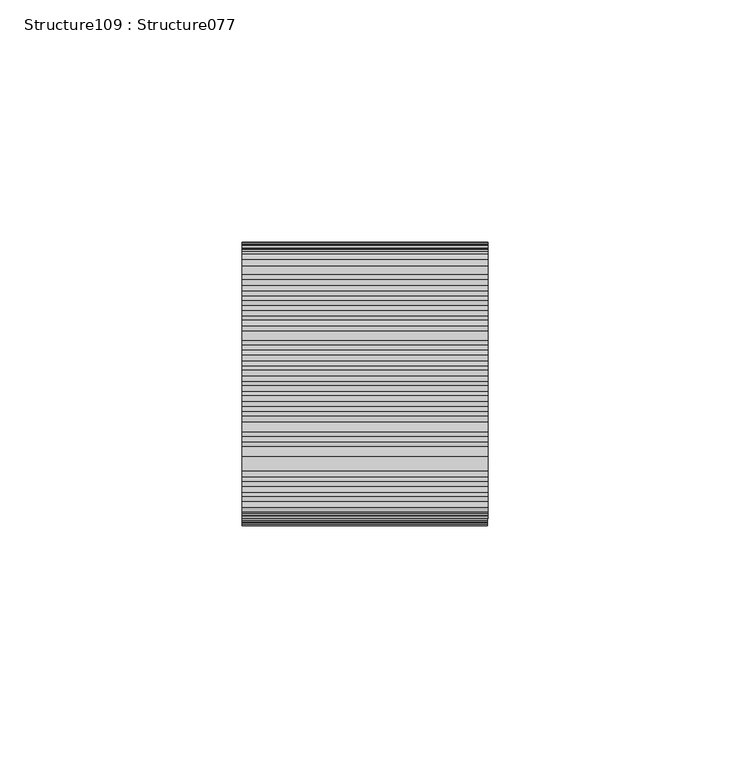
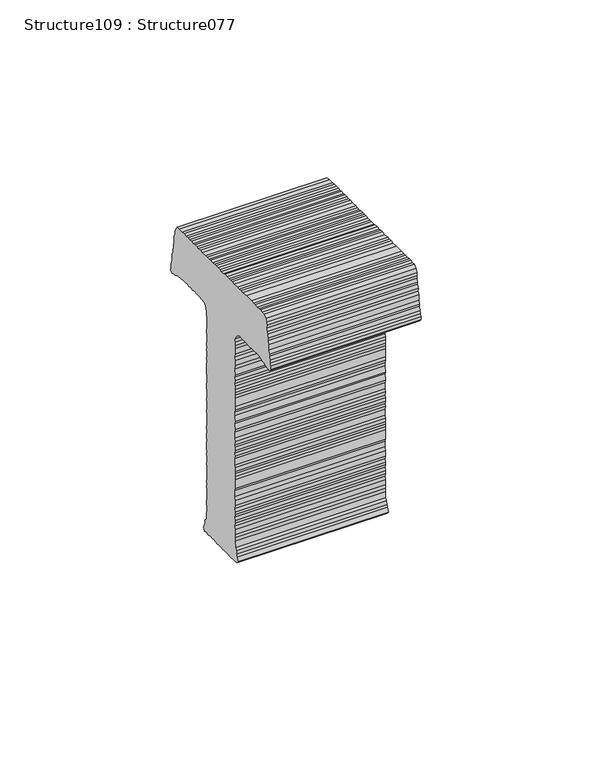
"""IFC4 building model written with IfcOpenShell, lengths in millimetres: proxy geometry, Structure109 : Structure077."""

from ifc_helpers import new_model, si_unit, frame, origin, place, context, project, spatial, polyline, outline, extrude, source, transform, mapped, element, save


def structure109_structure077_04282f25(model_context):
    return source(origin(), model_context, "Body", "SweptSolid", [
        extrude(outline(polyline([(1.289959, 0.0), (2.4826398, -0.634609), (3.3164572, -1.0932807), (3.9580093, -1.9186696), (4.9710555, -2.555887), (5.6151661, -3.0146845), (6.7250256, -3.5599982), (7.3660728, -4.3848855), (8.472829, -4.7530822), (9.8531305, -6.1242604), (10.9554405, -6.6690959), (11.5100349, -7.2200247), (12.6129687, -7.9530557), (13.4427489, -8.4082184), (14.2725291, -8.8633811), (15.1037896, -9.6891473), (15.1944421, -10.698522), (14.1870202, -11.5298818), (13.2730325, -12.0849252), (12.3559164, -12.4553038), (11.5300277, -13.0978639), (10.7973441, -13.4709018), (9.0493141, -14.4858701), (8.3217174, -15.4066268), (7.7726498, -16.1431226), (6.9457747, -16.7917245), (6.1253802, -17.8013525), (5.4844272, -18.4465702), (4.5633947, -19.001637), (3.7416407, -19.8288587), (3.2853709, -20.4764833), (2.2751721, -21.3050846), (1.543944, -22.0411781), (1.0973356, -24.1608888), (1.6488975, -25.9977611), (2.4780178, -26.6333239), (3.3998042, -27.367962), (4.0491583, -28.1940798), (5.4307221, -29.5665119), (6.2585694, -30.5769647), (7.1799825, -31.1231547), (8.4699132, -32.4045593), (9.2069822, -33.5058896), (10.7732057, -34.8736837), (11.2367929, -35.5222839), (12.2485769, -36.1582475), (12.8912362, -37.1657919), (13.6346844, -37.5351933), (14.4614986, -38.5375982), (15.2886229, -39.1781998), (15.9366173, -39.8219112), (16.6745753, -40.7360473), (18.7947568, -42.8422151), (19.7140189, -43.5743455), (20.1741694, -44.4005875), (21.0044202, -45.2253507), (22.6654609, -46.5062796), (23.0352406, -47.2427481), (24.6922424, -48.5196647), (25.2470551, -49.4399433), (26.8111276, -50.9936778), (27.6447916, -51.6337544), (28.4723865, -52.6439564), (29.1169786, -53.0962108), (30.038765, -53.8308488), (30.5895388, -54.7471151), (31.332832, -55.2974182), (31.9756463, -56.1240609), (33.5424955, -57.6805538), (34.2814973, -58.2265939), (35.2908779, -59.0482471), (35.8480941, -59.782836), (36.4905351, -60.4210307), (37.3206885, -61.0646414), (39.6269128, -63.3556224), (40.0845389, -64.1793567), (41.5610173, -65.646076), (42.5766853, -66.4669536), (43.9585014, -67.8396364), (44.6000535, -68.6650253), (45.523991, -69.2137229), (46.1692087, -69.854676), (46.7214971, -70.7724469), (47.6467942, -71.5035509), (48.3821304, -72.2340268), (49.0277214, -73.0634279), (49.9502418, -73.7917735), (51.2404249, -75.0734289), (52.0662869, -75.7127767), (52.8989071, -76.7209493), (54.5549225, -78.0039076), (55.4788926, -78.1830031), (56.4913023, -79.0076656), (57.2264202, -79.3687917), (58.6082305, -79.8291689), (58.7026461, -80.8352603), (57.9676565, -81.5751403), (57.3267991, -82.4010073), (56.50542, -83.4171802), (55.9549928, -83.9712697), (55.1291024, -84.6133267), (53.6628846, -86.0893001), (52.935542, -87.0108108), (52.1058902, -87.6566542), (51.2838854, -88.4841283), (50.7378453, -89.2231301), (49.9083484, -89.6880719), (49.1771203, -90.4241653), (48.4419756, -91.3449471), (47.7141624, -91.8968573), (47.1679673, -92.8167607), (46.0633822, -93.558621), (45.4222741, -94.3847406), (44.2272873, -94.1169737), (43.8574103, -93.1993527), (43.5804608, -92.0044109), (42.6585769, -91.0886203), (42.5601224, -90.0785165), (40.9893892, -88.3371098), (40.6233961, -87.6044028), (39.7960195, -86.9635506), (38.8722369, -86.2339511), (38.2270192, -85.592998), (37.4927269, -84.4944262), (36.8448298, -84.0318672), (36.0162486, -83.0277069), (35.3672443, -82.3829923), (34.4470933, -81.8380561), (33.8989413, -81.1054499), (33.0652772, -80.4653733), (32.5145035, -79.549107), (29.3755039, -76.4308552), (28.6416482, -76.0709829), (27.9988339, -75.2443402), (27.0731636, -74.3247882), (26.2422762, -73.6874699), (25.6009766, -72.8623318), (24.9520932, -72.4058145), (23.3854964, -70.8495724), (22.7428371, -69.8420279), (21.821424, -69.2958379), (21.1736819, -68.6523772), (20.5308676, -67.8257344), (19.6096094, -67.0986426), (18.3179459, -65.4463837), (17.5794256, -64.8938004), (16.7509417, -64.0707925), (16.2921742, -63.4340016), (15.090056, -62.6089619), (14.6310127, -61.9648754), (13.9887267, -61.1457791), (12.9725304, -60.3173552), (12.3279384, -59.8651009), (11.6784635, -58.8507858), (10.945749, -58.30397), (10.2991717, -57.4806107), (9.280572, -56.8378764), (8.4536027, -56.0163732), (7.9067128, -55.2850208), (7.2560966, -54.4576492), (6.6108788, -53.8166961), (5.6869413, -53.2679984), (3.4748744, -51.0705525), (2.740582, -49.9719806), (1.9113067, -49.5173194), (1.3560867, -48.7776919), (0.620498, -48.0469653), (-0.2129136, -47.4071394), (-0.7654545, -46.4891177), (-1.6823238, -45.9474415), (-2.3317988, -44.9331264), (-3.1594278, -44.2920234), (-3.8950165, -43.5612967), (-4.8203136, -42.8301927), (-6.1079382, -41.181946), (-6.9378391, -40.538586), (-7.3981213, -39.9002905), (-8.3199077, -39.1656525), (-9.1505426, -38.528585), (-9.7955079, -37.8878827), (-11.5384176, -36.8807156), (-12.4611829, -37.0649281), (-13.8384528, -37.8980173), (-14.8461289, -38.7286231), (-15.3965561, -39.2827127), (-16.0358988, -40.1100843), (-16.9497891, -40.8462803), (-17.5928932, -41.6774383), (-18.6009408, -42.3200993), (-19.0556003, -43.1498778), (-19.8825962, -43.6102823), (-20.612344, -44.7169794), (-21.3486932, -45.2744531), (-23.1741727, -47.6684522), (-23.7231446, -48.5855974), (-24.1776816, -49.6040764), (-24.6342272, -50.2444054), (-25.1856026, -51.3472402), (-26.2867062, -51.166216), (-26.7507747, -50.5241591), (-27.5782488, -49.7021543), (-28.1285194, -48.7858863), (-28.5969769, -47.9584139), (-29.4239461, -47.1369107), (-30.1573836, -46.2202437), (-30.4442844, -45.2110164), (-30.9911743, -44.479664), (-31.5499051, -43.7435706), (-32.286756, -43.0115901), (-32.7467531, -42.0039433), (-33.6726759, -41.0841405), (-34.3148645, -40.4461966), (-34.684839, -39.3474231), (-35.5160995, -38.5216569), (-35.9848061, -36.4049811), (-35.1593865, -35.3933237), (-33.877731, -34.1031405), (-33.2381375, -33.2755165), (-32.3207366, -32.5357865), (-31.5906172, -31.6170343), (-30.7675037, -30.972219), (-30.2149253, -30.232189), (-29.3014407, -29.6771472), (-28.7522182, -28.7597496), (-27.9267027, -27.9287414), (-27.1977806, -27.5594901), (-26.4604849, -26.452768), (-25.5467496, -25.8974738), (-24.2649393, -24.4263889), (-23.533866, -23.8711972), (-22.7988764, -23.1313173), (-22.2496538, -22.2139197), (-21.3360143, -21.4779761), (-20.6929102, -20.646818), (-20.0522078, -20.0018527), (-19.1383176, -19.2656567), (-18.3128021, -18.4346486), (-17.6722547, -17.970585), (-16.7597241, -17.0519827), (-16.3880425, -16.3133074), (-15.4757627, -15.3949576), (-14.6488875, -14.7463557), (-14.009294, -13.9187316), (-13.3685917, -13.2737663), (-12.3608199, -12.6238099), (-11.0803691, -10.9703188), (-10.3440199, -10.4128451), (-9.6141513, -9.4943453), (-8.7909419, -9.0301793), (-7.5104911, -7.3766882), (-5.3998096, -5.2519629), (-4.3918828, -4.4211047), (-3.7546911, -3.7796734), (-2.9293306, -3.1295671), (-2.1976967, -2.2123194), (-1.6488799, -1.476076), (-0.7316338, -0.9172476), (0.0, 0.0), (1.289959, 0.0)])), frame((-56111.5642738, 291173.858936, -276.594816), z_axis=(-0.9999998917542983, 0.0004652863545059615, 0.0), x_axis=(-0.0003279144188290442, -0.7047582207414732, -0.7094474911996285)), (0.0, 0.0, 1.0), 50.8),
    ])


if __name__ == "__main__":
    model = new_model("IFC4")
    model_context = context("Model", 3, world=origin())
    ifc_project = project(units=[si_unit("LENGTHUNIT", "METRE", prefix="MILLI")], contexts=[model_context])
    site = spatial("IfcSite", under=ifc_project)
    building = spatial("IfcBuilding", under=site)
    placement = place(None, origin())
    structure109_structure077_shape = structure109_structure077_04282f25(model_context)
    element("IfcBuildingElementProxy", 1, Name="Structure109 : Structure077", ObjectType="Structure109 : Structure077", at=placement, inside=building, context=model_context, shape_type="MappedRepresentation", body=[
        mapped(structure109_structure077_shape, transform((0.0, 0.0, 0.0), x_axis=(1.0, 0.0, 0.0), y_axis=(0.0, 1.0, 0.0), z_axis=(0.0, 0.0, 1.0))),
    ])
    save(model, "model.ifc")

# Revit data of these elements
# Type "Structure109 : Structure077"
#   NameOverride = "Structure077"
# Element 1 (IfcBuildingElementProxy, "Structure109 : Structure077")
#   Materials on its faces: "BRUSHED ALUMINUM LETTERING"
# Materials
#   "BRUSHED ALUMINUM LETTERING": class "Unassigned", colour RGB 169 181 186, transparency 0, Cost = 0
